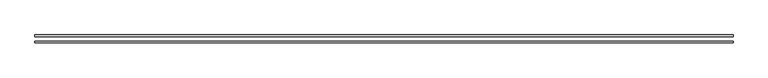
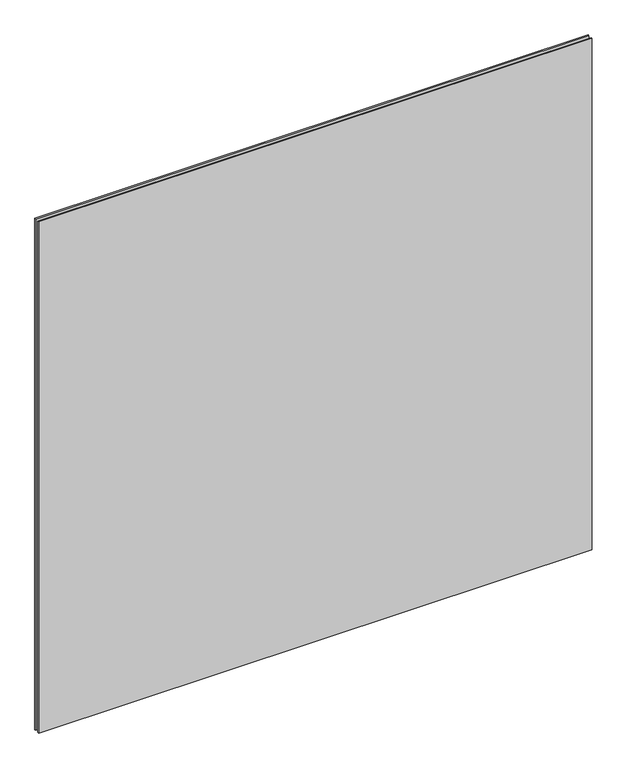
"""IFC4 building model written with IfcOpenShell, lengths in millimetres: proxy geometry, Window glass001 499 : Window glass001 499."""

from ifc_helpers import new_model, si_unit, frame, origin, place, context, project, spatial, polyline, outline, extrude, source, transform, mapped, element, save


def generic_models_bfa8a63e(model_context):
    return source(origin(), model_context, "Body", "SweptSolid", [
        extrude(outline(polyline([(3694.2883192, 9729.8604245), (3694.2883192, 9734.6229245), (5694.2883192, 9734.6229245), (5694.2883192, 9729.8604245), (3694.2883192, 9729.8604245)])), frame((0.0, 0.0, 37537.6466125), z_axis=(0.0, 0.0, 1.0), x_axis=(1.0, 0.0, 0.0)), (0.0, 0.0, 1.0), 1951.99),
        extrude(outline(polyline([(3694.2883192, 9747.6404245), (3694.2883192, 9752.4029245), (5694.2883192, 9752.4029245), (5694.2883192, 9747.6404245), (3694.2883192, 9747.6404245)])), frame((0.0, 0.0, 37537.6466125), z_axis=(0.0, 0.0, 1.0), x_axis=(1.0, 0.0, 0.0)), (0.0, 0.0, 1.0), 1951.99),
    ])


if __name__ == "__main__":
    model = new_model("IFC4")
    model_context = context("Model", 3, world=origin())
    ifc_project = project(units=[si_unit("LENGTHUNIT", "METRE", prefix="MILLI")], contexts=[model_context])
    site = spatial("IfcSite", under=ifc_project)
    building = spatial("IfcBuilding", under=site)
    placement = place(None, origin())
    generic_models_shape = generic_models_bfa8a63e(model_context)
    element("IfcBuildingElementProxy", 1, Name="Window glass001 499 : Window glass001 499", ObjectType="Window glass001 499 : Window glass001 499", at=placement, inside=building, context=model_context, shape_type="MappedRepresentation", body=[
        mapped(generic_models_shape, transform((0.0, 0.0, 0.0), x_axis=(1.0, 0.0, 0.0), y_axis=(0.0, 1.0, 0.0), z_axis=(0.0, 0.0, 1.0))),
    ])
    save(model, "model.ifc")

# Revit data of these elements
# Type "Window glass001 499 : Window glass001 499"
#   NameOverride = "Window glass001"
# Element 1 (IfcBuildingElementProxy, "Window glass001 499 : Window glass001 499")
#   Materials on its faces: "1\"  INSULATED GLAZING"
# Materials
#   "1\"  INSULATED GLAZING": class "Unassigned", colour RGB 146 199 212, transparency 0, Cost = 0
